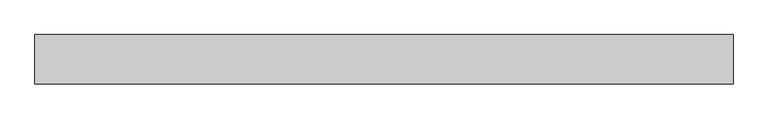
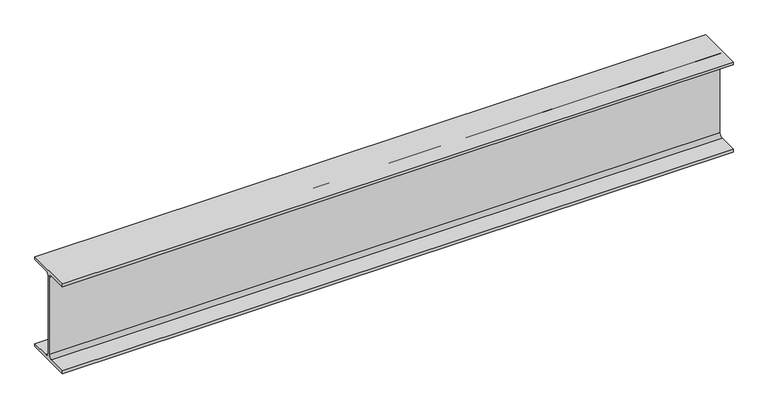
"""IFC4 building model written with IfcOpenShell, lengths in millimetres: beam geometry, 0912_Steel Framing_H-KSD3502 : H_SB_ASB_H-350x175x7x11."""

from ifc_helpers import new_model, si_unit, point, frame, frame_2d, origin, place, context, project, spatial, polyline, circle_curve, trimmed, segment, composite_curve, outline, extrude, source, transform, mapped, element, save


def beam_172b79b6(model_context):
    return source(origin(), model_context, "Body", "SweptSolid", [
        extrude(outline(composite_curve([segment(polyline([(87.5, -164.0), (87.5, -175.0), (-87.5, -175.0), (-87.5, -164.0), (-17.5, -164.0)]), True, "CONTINUOUS"), segment(trimmed(circle_curve(frame_2d((-17.5, -150.0)), 14.0), [point((-17.5, -164.0))], [point((-3.5, -150.0))], True, "CARTESIAN"), True, "CONTINUOUS"), segment(polyline([(-3.5, -150.0), (-3.5, 150.0)]), True, "CONTINUOUS"), segment(trimmed(circle_curve(frame_2d((-17.5, 150.0)), 14.0), [point((-3.5, 150.0))], [point((-17.5, 164.0))], True, "CARTESIAN"), True, "CONTINUOUS"), segment(polyline([(-17.5, 164.0), (-87.5, 164.0), (-87.5, 175.0), (87.5, 175.0), (87.5, 164.0), (17.5, 164.0)]), True, "CONTINUOUS"), segment(trimmed(circle_curve(frame_2d((17.5, 150.0)), 14.0), [point((17.5, 164.0))], [point((3.5, 150.0))], True, "CARTESIAN"), True, "CONTINUOUS"), segment(polyline([(3.5, 150.0), (3.5, -150.0)]), True, "CONTINUOUS"), segment(trimmed(circle_curve(frame_2d((17.5, -150.0)), 14.0), [point((3.5, -150.0))], [point((17.5, -164.0))], True, "CARTESIAN"), True, "CONTINUOUS"), segment(polyline([(17.5, -164.0), (87.5, -164.0)]), True, "CONTINUOUS")], self_intersect=False)), frame((-1175.6379608, 0.0, 0.0), z_axis=(1.0, 0.0, 0.0), x_axis=(0.0, 1.0, 0.0)), (0.0, 0.0, 1.0), 2471.4118659),
    ])


if __name__ == "__main__":
    model = new_model("IFC4")
    model_context = context("Model", 3, world=origin())
    ifc_project = project(units=[si_unit("LENGTHUNIT", "METRE", prefix="MILLI")], contexts=[model_context])
    site = spatial("IfcSite", under=ifc_project)
    building = spatial("IfcBuilding", under=site)
    placement = place(None, origin())
    beam_shape = beam_172b79b6(model_context)
    element("IfcBeam", 1, ObjectType="0912_Steel Framing_H-KSD3502 : H_SB_ASB_H-350x175x7x11", at=placement, inside=building, context=model_context, shape_type="MappedRepresentation", body=[
        mapped(beam_shape, transform((0.0, 0.0, 0.0), x_axis=(1.0, 0.0, 0.0), y_axis=(0.0, 1.0, 0.0), z_axis=(0.0, 0.0, 1.0))),
    ])
    save(model, "model.ifc")

# Revit data of these elements
# Type "0912_Steel Framing_H-KSD3502 : H_SB_ASB_H-350x175x7x11"
#   H_WM Code_1 = "S01AA002-00001 | Main Steel Structure Fabrication Work | Shelter/Building | Medium Steel - Standard (90KG/M>Weight≥30KG/M) | Material: (   )"
#   H_WM Code_2 = "S03AA028-00001 | Main Steel Structure Erection Work | Shelter/Building | Medium Steel (90KG/M>Weight≥30KG/M) | Material: (   )"
#   H_WM Code_3 = "S01AA010-00001 | Main Steel Structure Fabrication Work | Shelter/Building | Steel Painting/Coating | for Non-Fireproofed Steel Surface, Surface Preparation, Primer, Second & Final Coat | Material: (   )"
#   H_Q'ty Cal Type Tag = "SB-Q2"
#   Width = 17.5 cm
#   Web Thickness = 0.7 cm
#   Web Fillet = 1.4 cm
#   Warping Constant = 282000.0 cm⁶
#   W = 0
#   Torsional Moment of Inertia = 19.4042 cm⁴
#   Section Area = 63.14 cm²
#   Plastic Modulus weak axis = 174.0 cm³
#   Plastic Modulus strong axis = 868.0 cm³
#   Perimeter = 1.36 m²/m
#   Nominal Weight = 49.60 kgf/m
#   Moment of Inertia weak axis = 984.00 cm⁴
#   Moment of Inertia strong axis = 13600.00 cm⁴
#   Height = 35.0 cm
#   Flange Thickness = 1.1 cm
#   Elastic Modulus weak axis = 112.0 cm³
#   Elastic Modulus strong axis = 775.0 cm³
#   Centroid Vertical = 17.5 cm
#   Centroid Horizontal = 8.75 cm
#   Ix = 136000000
#   Length [instance default] = 1.5240 m
#   Zx = 868000
#   b = 0.1750 m
#   h = 0.3500 m
#   r = 0.0140 m
#   s = 0.0070 m
#   t = 0.0110 m
#   A = 0.006314 m²
#   Structural Material [instance default] = Steel, 45-345
#   Assembly Code = ""
# Element 1 (IfcBeam, "0912_Steel Framing_H-KSD3502 : H_SB_ASB_H-350x175x7x11")
#   Structural Material = none
# Materials
#   "Steel, 45-345": class "Metal", colour RGB 189 187 185, transparency 0, Description = "Steel 345 MPa", Cost = 0
